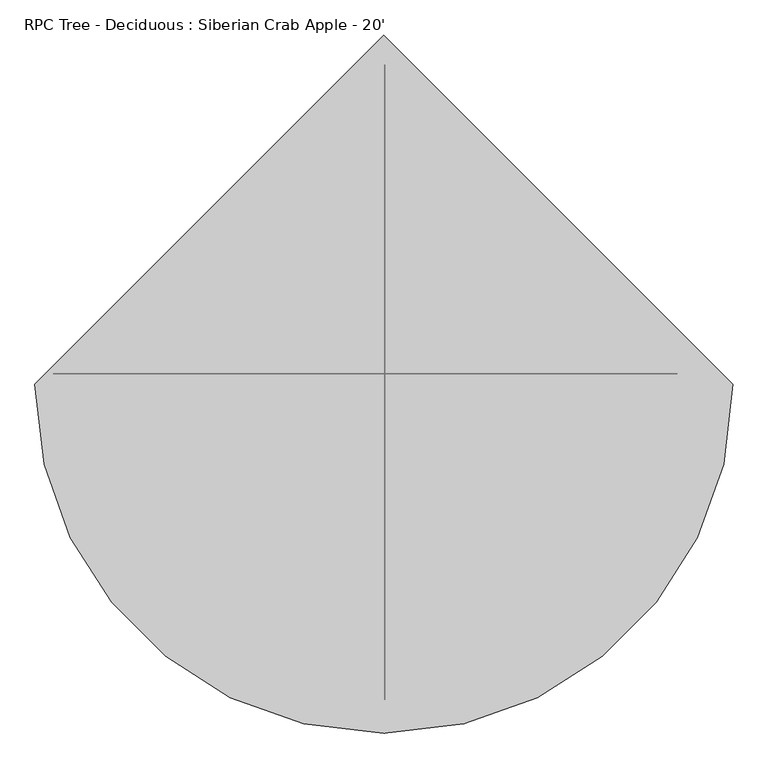
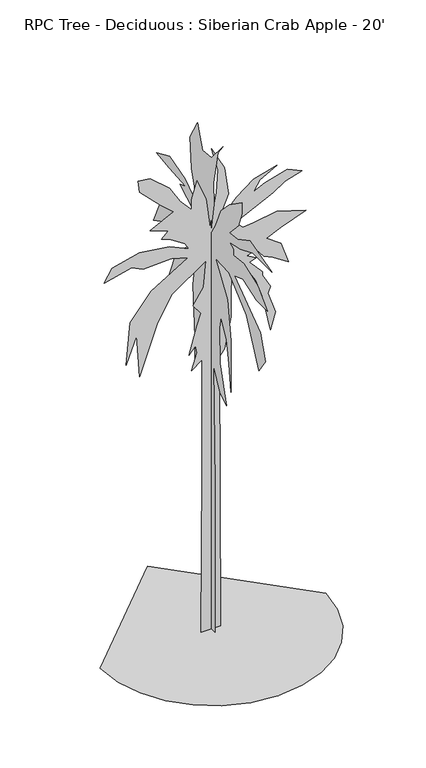
"""IFC4 building model written with IfcOpenShell, lengths in millimetres: geographic element geometry, RPC Tree - Deciduous : Siberian Crab Apple - 20'."""

from ifc_helpers import new_model, si_unit, origin, place, context, project, spatial, triangles, source, transform, mapped, element, save


def rpc_tree_deciduous_siberian_crab_apple_20_db2ab023(model_context):
    return source(origin(), model_context, "Body", "Tessellation", [
        triangles([(-43.5060926, -0.0139928, 0.000755), (-120.0335708, -0.0139996, 0.0007583), (-104.7279553, -0.0143505, 1995.7187359), (-104.7277554, -0.0145941, 3357.8970726), (-227.1712718, -0.0145724, 3266.0709915), (-165.9502267, -0.0146106, 3465.0443115), (-181.2552336, -0.0146263, 3556.8701019), (-257.7833204, -0.0146066, 3465.0443115), (-165.9500268, -0.0146708, 3801.7664909), (-120.033371, -0.0146974, 3939.515641), (-211.8662649, -0.0147153, 4061.9639809), (-89.4225396, -0.0147535, 4245.6158524), (-58.8115083, -0.0148123, 4567.0372215), (-456.754533, -0.0147457, 4291.539212), (-625.1136606, -0.0146863, 4000.7398109), (-839.3919331, -0.0145702, 3403.8201416), (-870.0019833, -0.0146619, 3924.2148308), (-992.4461082, -0.0145991, 3602.7934616), (-946.5311056, -0.0146914, 4107.8667023), (-701.642783, -0.0147569, 4413.9872612), (-273.0883274, -0.0148221, 4674.1847511), (-472.0595581, -0.0148244, 4735.4086304), (-793.4748957, -0.0148076, 4720.0874725), (-931.2240458, -0.0148125, 4781.3116425), (-1252.6393833, -0.0147848, 4704.7863716), (-1160.8072706, -0.0148162, 4857.8366226), (-839.3919331, -0.0148439, 4934.3819504), (-487.3645469, -0.0148511, 4888.4585907), (-257.7833204, -0.014842, 4781.3116425), (-303.700376, -0.0148536, 4857.8366226), (-487.3645469, -0.0148675, 4980.2849625), (-579.198658, -0.014869, 5010.9069305), (-502.6716067, -0.014886, 5087.4319107), (-716.9478081, -0.0148903, 5163.9568909), (-441.4495442, -0.014927, 5301.706041), (-594.5036831, -0.0149449, 5439.455191), (-839.3919331, -0.014978, 5684.3518707), (-854.6969582, -0.015002, 5822.1010208), (-716.9478081, -0.0150052, 5806.779863), (-487.3645469, -0.0149797, 5607.806543), (-364.9204219, -0.0149495, 5408.833223), (-227.1712718, -0.0149281, 5255.7832626), (-227.1712718, -0.01495, 5378.2310211), (-165.9500268, -0.014991, 5592.5057327), (-58.8115083, -0.0149492, 5332.3082428), (-12.8950795, -0.0148855, 4964.9835709), (63.6324214, -0.01496, 5362.9302109), (78.9380414, -0.0150099, 5638.428511), (2.4105388, -0.0150586, 5929.2276215), (155.4655287, -0.0150133, 5638.428511), (201.3821664, -0.0149551, 5301.706041), (63.6324214, -0.0148888, 4964.9835709), (293.2152783, -0.0149454, 5225.1810608), (492.1864909, -0.0149815, 5378.2310211), (767.6847548, -0.0150072, 5454.7565826), (568.7135422, -0.0149793, 5347.6294006), (492.1864909, -0.0149541, 5225.1810608), (629.9356047, -0.0149711, 5286.4052307), (890.1288797, -0.0149961, 5362.9302109), (1058.4901148, -0.0149898, 5286.4052307), (859.5189022, -0.0149702, 5225.1810608), (721.7697521, -0.0149477, 5133.3349228), (277.9102714, -0.01489, 4919.0607925), (369.7423659, -0.0148776, 4827.2347115), (492.1864909, -0.0148857, 4842.5355217), (767.6847548, -0.0149059, 4888.4585907), (1104.4071522, -0.0149015, 4781.3116425), (813.6017921, -0.0148696, 4674.1847511), (645.2406298, -0.0148486, 4597.6594803), (813.6017921, -0.0148341, 4475.2114311), (905.4339048, -0.0147915, 4215.0139412), (721.7697521, -0.0148054, 4337.462281), (614.6306522, -0.0148089, 4383.3650024), (492.1864909, -0.0148309, 4536.435601), (492.1864909, -0.0148227, 4490.5122414), (415.6594033, -0.0148139, 4459.9103302), (522.7965048, -0.0148077, 4398.686451), (446.2694172, -0.0147988, 4368.0641922), (599.3255908, -0.0147754, 4199.713131), (599.3255908, -0.0147672, 4153.790062), (691.1576672, -0.0147411, 3985.4390007), (660.5476896, -0.0147261, 3908.9137299), (752.3797297, -0.0146836, 3648.7165306), (691.1576672, -0.0146453, 3449.7432106), (599.3255908, -0.0147207, 3893.592572), (522.7965048, -0.0147584, 4123.1881508), (385.0473547, -0.0147934, 4352.7630913), (247.2982228, -0.0147984, 4413.9872612), (231.9932158, -0.0147429, 4107.8667023), (231.9932158, -0.0146827, 3771.1645798), (155.4655287, -0.0146137, 3403.8201416), (94.2434572, -0.0145973, 3327.2951614), (109.5488729, -0.0140041, 0.0007483), (-0.0029664, 71.6789324, 0.000396), (-0.0029667, 130.9067988, 0.0004066), (-0.0029664, 130.9067988, 1461.423151), (-0.0029648, 116.1000355, 3430.7440796), (-0.0029661, 175.3274886, 3341.9050255), (-0.0029645, 323.3965393, 3030.9484245), (-0.0029657, 323.3965393, 3401.1377472), (-0.0029655, 367.8180648, 4023.0308922), (-0.0029666, 308.5893763, 4452.432589), (-0.0029673, 427.0446822, 4319.1538055), (-0.0029654, 634.3430391, 3889.7521088), (-0.0029651, 871.253651, 3593.6289047), (-0.0029668, 1048.9356108, 3312.2989838), (-0.0029657, 841.639325, 3874.9591164), (-0.0029659, 708.3768196, 4200.7087097), (-0.0029659, 412.2375192, 4496.8522614), (-0.0029672, 545.5000245, 4467.2255814), (-0.0029658, 723.1839827, 4452.432589), (-0.0029661, 886.0608141, 4482.0389214), (-0.002966, 1167.3929878, 4333.9671455), (-0.002967, 1019.3233194, 4659.7167389), (-0.0029654, 856.446488, 4659.7167389), (-0.0029657, 797.2178358, 4911.4409088), (-0.0029661, 515.8876968, 4852.2078964), (-0.0029671, 338.2037024, 4941.0466599), (-0.0029672, 634.3430391, 5103.9320663), (-0.0029647, 515.8876968, 5148.3514481), (-0.0029665, 841.639325, 5177.9577805), (-0.0029651, 1108.1643356, 5207.5838791), (-0.0029658, 841.639325, 5326.0289749), (-0.002966, 530.6948599, 5237.1902115), (-0.0029674, 278.975032, 5059.5121033), (-0.0029656, 397.4323909, 5444.4949997), (-0.0029655, 427.0446822, 5814.6636841), (-0.0029661, 278.975032, 6081.1805557), (-0.0029655, 249.3627225, 5992.3417923), (-0.0029656, 175.3274886, 5799.8506348), (-0.0029669, -2.3556546, 5814.6636841), (-0.002965, -239.2657371, 6095.9941864), (-0.0029662, -135.6181846, 5962.7354599), (-0.0029667, -46.7763917, 5533.3337631), (-0.0029668, -61.5833549, 5281.6095932), (-0.0029672, 12.4512499, 4867.0212364), (-0.0029646, -91.1974948, 5029.8860046), (-0.0029668, -194.8458467, 5281.6095932), (-0.0029668, -372.5282061, 5459.2877014), (-0.0029672, -624.2460537, 5636.9861572), (-0.0029672, -624.2460537, 5503.7070831), (-0.0029666, -550.2122005, 5311.2362732), (-0.0029673, -372.5282061, 5118.7451157), (-0.0029651, -535.4050375, 5133.5378174), (-0.0029673, -787.1228851, 5266.7965439), (-0.0029659, -1231.3318176, 5148.3514481), (-0.0029665, -846.3515373, 5148.3514481), (-0.0029658, -594.633726, 5044.699054), (-0.0029667, -372.5282061, 5000.2796722), (-0.0029661, -446.5640576, 4955.8602905), (-0.0029664, -446.5640576, 4881.8345764), (-0.0029661, -668.6675428, 4911.4409088), (-0.0029656, -949.9997166, 4807.7885147), (-0.0029651, -1142.4888393, 4615.2973572), (-0.002967, -920.3853178, 4615.2973572), (-0.0029653, -639.0532167, 4704.1361206), (-0.0029665, -476.1784201, 4644.9237465), (-0.0029655, -994.4212057, 4259.9414314), (-0.0029657, -1098.069385, 3963.7981705), (-0.0029654, -964.8068796, 3771.3070129), (-0.0029657, -713.089032, 4304.3611038), (-0.0029655, -357.7230778, 4615.2973572), (-0.0029648, -91.1974948, 4630.1106972), (-0.0029653, -328.1087517, 4259.9414314), (-0.0029655, -402.1425685, 3800.9130547), (-0.0029673, -402.1425685, 3164.2272079), (-0.0029656, -357.7230778, 3489.9768013), (-0.0029664, -313.3015886, 3756.4936729), (-0.0029666, -194.8458467, 3963.7981705), (-0.002966, -165.2319202, 3815.7263947), (-0.0029652, -180.0388834, 3386.3246979), (-0.0029673, -313.3015886, 2942.1096611), (-0.0029663, -180.0388834, 3030.9484245), (-0.0029668, -46.7763917, 3282.6723038), (-0.0029651, -76.3905225, 1831.5961956), (-0.0029671, -76.3905225, 0.0003695), (-1322.4771263, -39.3033105, 0.0004339), (-1287.6100685, -341.4996131, 0.0003784), (-1188.3103884, -619.0197012, 0.0003244), (-1032.5292721, -863.9120934, 0.0002738), (-828.2179785, -1068.223387, 0.0002283), (-583.325659, -1224.0045033, 0.0001898), (-305.8075693, -1323.3041107, 0.0001599), (-3.6097429, -1358.1711685, 0.0001404), (298.5878792, -1323.3041107, 0.0001335), (576.1059689, -1224.0045033, 0.0001391), (820.9982883, -1068.223387, 0.0001562), (1025.3095819, -863.9120934, 0.0001838), (1181.0906982, -619.0197012, 0.0002208), (1280.3903057, -341.4996131, 0.0002661), (1315.2573635, -39.3033105, 0.0003186), (-3.6099867, 1279.5633213, 0.0002422)], [[54, 55, 56], [48, 49, 50], [17, 18, 19], [15, 16, 17], [7, 8, 9], [83, 84, 85], [82, 83, 85], [4, 5, 6], [70, 71, 72], [66, 67, 68], [43, 44, 45], [59, 60, 61], [24, 25, 26], [24, 26, 27], [33, 34, 35], [76, 77, 78], [58, 59, 61], [58, 61, 62], [31, 32, 33], [42, 43, 45], [42, 45, 46], [37, 38, 39], [54, 56, 57], [53, 54, 57], [23, 24, 27], [23, 27, 28], [22, 23, 28], [22, 28, 29], [21, 22, 29], [58, 62, 63], [57, 58, 63], [53, 57, 63], [52, 53, 63], [36, 37, 39], [36, 39, 40], [36, 40, 41], [35, 36, 41], [35, 41, 42], [69, 70, 72], [69, 72, 73], [69, 73, 74], [65, 66, 68], [65, 68, 69], [65, 69, 74], [64, 65, 74], [47, 48, 50], [47, 50, 51], [46, 47, 51], [46, 51, 52], [33, 35, 42], [82, 85, 86], [81, 82, 86], [80, 81, 86], [33, 42, 46], [31, 33, 46], [30, 31, 46], [29, 30, 46], [15, 17, 19], [15, 19, 20], [14, 15, 20], [14, 20, 21], [13, 14, 21], [92, 93, 1], [92, 1, 2], [92, 2, 3], [92, 3, 4], [80, 86, 87], [79, 80, 87], [78, 79, 87], [76, 78, 87], [76, 87, 88], [13, 21, 29], [13, 29, 46], [13, 46, 52], [13, 52, 63], [13, 63, 64], [13, 64, 74], [13, 74, 75], [13, 75, 76], [13, 76, 88], [12, 13, 88], [12, 88, 89], [11, 12, 89], [10, 11, 89], [10, 89, 90], [9, 10, 90], [9, 90, 91], [7, 9, 91], [6, 7, 91], [4, 6, 91], [92, 4, 91], [131, 132, 133], [165, 166, 167], [105, 106, 107], [145, 146, 147], [165, 167, 168], [98, 99, 100], [131, 133, 134], [121, 122, 123], [104, 105, 107], [112, 113, 114], [171, 172, 173], [171, 173, 174], [153, 154, 155], [127, 128, 129], [118, 119, 120], [112, 114, 115], [139, 140, 141], [139, 141, 142], [159, 160, 161], [158, 159, 161], [157, 158, 161], [157, 161, 162], [104, 107, 108], [103, 104, 108], [103, 108, 109], [102, 103, 109], [127, 129, 130], [121, 123, 124], [120, 121, 124], [120, 124, 125], [118, 120, 125], [153, 155, 156], [152, 153, 156], [151, 152, 156], [151, 156, 157], [126, 127, 130], [145, 147, 148], [144, 145, 148], [144, 148, 149], [143, 144, 149], [139, 142, 143], [138, 139, 143], [137, 138, 143], [137, 143, 149], [175, 176, 94], [175, 94, 95], [175, 95, 96], [175, 96, 97], [174, 175, 97], [111, 112, 115], [115, 116, 117], [111, 115, 117], [110, 111, 117], [109, 110, 117], [165, 168, 169], [164, 165, 169], [130, 131, 134], [126, 130, 134], [126, 134, 135], [125, 126, 135], [125, 135, 136], [118, 125, 136], [151, 157, 162], [171, 174, 97], [170, 171, 97], [109, 117, 118], [109, 118, 136], [102, 109, 136], [97, 98, 100], [97, 100, 101], [170, 97, 101], [169, 170, 101], [169, 101, 102], [164, 169, 102], [163, 164, 102], [163, 102, 136], [151, 162, 163], [151, 163, 136], [151, 136, 137], [151, 137, 149], [151, 149, 150], [191, 192, 177], [190, 191, 177], [190, 177, 178], [189, 190, 178], [189, 178, 179], [189, 179, 180], [188, 189, 180], [187, 188, 180], [187, 180, 181], [187, 181, 182], [187, 182, 183], [187, 183, 184], [187, 184, 185], [187, 185, 186]], closed=False),
    ])


if __name__ == "__main__":
    model = new_model("IFC4")
    model_context = context("Model", 3, world=origin())
    ifc_project = project(units=[si_unit("LENGTHUNIT", "METRE", prefix="MILLI")], contexts=[model_context])
    site = spatial("IfcSite", under=ifc_project)
    building = spatial("IfcBuilding", under=site)
    placement = place(None, origin())
    rpc_tree_deciduous_siberian_crab_apple_20_shape = rpc_tree_deciduous_siberian_crab_apple_20_db2ab023(model_context)
    element("IfcGeographicElement", 1, ObjectType="RPC Tree - Deciduous : Siberian Crab Apple - 20'", at=placement, inside=building, context=model_context, shape_type="MappedRepresentation", body=[
        mapped(rpc_tree_deciduous_siberian_crab_apple_20_shape, transform((0.0, 0.0, 0.0), x_axis=(1.0, 0.0, 0.0), y_axis=(0.0, 1.0, 0.0), z_axis=(0.0, 0.0, 1.0))),
    ])
    save(model, "model.ifc")

# Revit data of these elements
# Type "RPC Tree - Deciduous : Siberian Crab Apple - 20'"
#   built-in parameter 1005195 = "RPC-16-FVGV-NKG0-7NHH-C000-ST1L-LVER-AU"
#   Type Comments = "Siberian Crab Apple"
#   Assembly Code = "G2050500"
#   Height = 6.096 m
#   Default Elevation = 0
